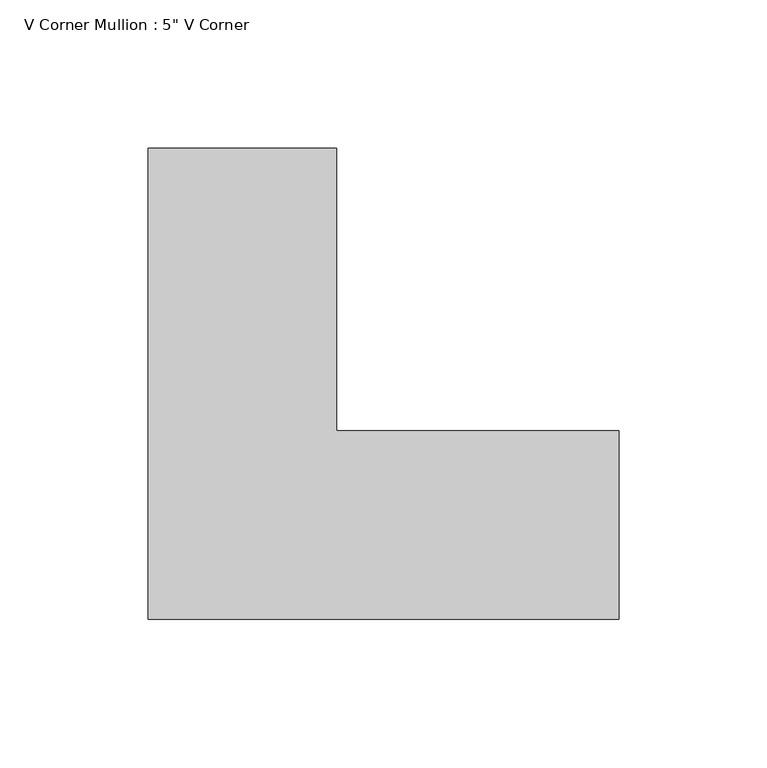
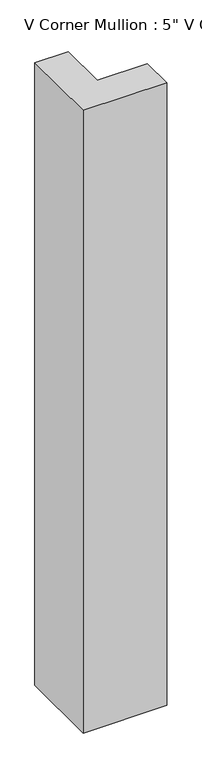
"""IFC4 building model written with IfcOpenShell, lengths in millimetres: member geometry."""

import ifcopenshell
import ifcopenshell.guid

model = None  # the IFC model being written
_history = None  # IfcOwnerHistory: only IFC2X3 demands one
_inside = {}  # id of a spatial element -> (the spatial element, [elements in it])
_under = {}  # id of a project, library or spatial element -> (it, [spatial elements below it])
_declared = {}  # id of a project -> (the project, [libraries it declares])
_typed = {}  # id of a type object -> (the type object, [elements of that type])
_made_of = {}  # id of a material, layer set ... -> (it, [elements and type objects made of it])


def new_model(schema):
    """Start an empty IFC model of exactly this schema.

    Asked for "IFC4X3", IfcOpenShell would pick the latest addendum, in which some entities
    have other attributes; the version numbers below select the first issue.
    IFC2X3 requires an IfcOwnerHistory on every rooted entity: one is made here for all.
    """
    global model, _history
    if schema == "IFC4X3":
        model = ifcopenshell.file(schema_version=(4, 3, 0, 0))
    else:
        model = ifcopenshell.file(schema=schema)
    _inside.clear()
    _under.clear()
    _declared.clear()
    _typed.clear()
    _made_of.clear()
    _history = None
    if model.schema == "IFC2X3":
        org = make("IfcOrganization", Name="unknown")
        user = make(
            "IfcPersonAndOrganization",
            ThePerson=make("IfcPerson", FamilyName="unknown"),
            TheOrganization=org,
        )
        app = make(
            "IfcApplication",
            ApplicationDeveloper=org,
            Version="unknown",
            ApplicationFullName="unknown",
            ApplicationIdentifier="unknown",
        )
        _history = make(
            "IfcOwnerHistory",
            OwningUser=user,
            OwningApplication=app,
            ChangeAction="ADDED",
            CreationDate=0,
        )
    return model


def make(cls, **values):
    """One entity of the class cls with the attributes given. An attribute that is None is left unset."""
    return model.create_entity(
        cls, **{name: value for name, value in values.items() if value is not None}
    )


def rooted(cls, **values):
    """An entity with a GlobalId (a new one), such as an element, a storey or a relation."""
    return make(cls, GlobalId=ifcopenshell.guid.new(), OwnerHistory=_history, **values)


def si_unit(unit_type, name, prefix=None):
    """IfcSIUnit, for example si_unit("LENGTHUNIT", "METRE", prefix="MILLI")."""
    return make("IfcSIUnit", UnitType=unit_type, Prefix=prefix, Name=name)


def assignment(units):
    """IfcUnitAssignment: the units of a project."""
    return None if units is None else make("IfcUnitAssignment", Units=units)


def point(xyz):
    """IfcCartesianPoint."""
    return None if xyz is None else make("IfcCartesianPoint", Coordinates=xyz)


def direction(xyz):
    """IfcDirection."""
    return None if xyz is None else make("IfcDirection", DirectionRatios=xyz)


def frame(location, z_axis=None, x_axis=None):
    """IfcAxis2Placement3D, a coordinate frame: its origin and axes. An axis left out is left unset."""
    return make(
        "IfcAxis2Placement3D",
        Location=point(location),
        Axis=direction(z_axis),
        RefDirection=direction(x_axis),
    )


def origin():
    """The frame at (0, 0, 0) with its axes left unset."""
    return frame((0.0, 0.0, 0.0))


def place(relative_to, where):
    """IfcLocalPlacement: puts the frame where relative to a parent placement (None: the world)."""
    return make(
        "IfcLocalPlacement", PlacementRelTo=relative_to, RelativePlacement=where
    )


def context(
    kind, dimensions, precision=None, world=None, true_north=None, identifier=None
):
    """IfcGeometricRepresentationContext, for example the 3D "Model" context."""
    return make(
        "IfcGeometricRepresentationContext",
        ContextIdentifier=identifier,
        ContextType=kind,
        CoordinateSpaceDimension=dimensions,
        Precision=precision,
        WorldCoordinateSystem=world,
        TrueNorth=true_north,
    )


def project(units=None, contexts=None):
    """IfcProject with its units and contexts."""
    return rooted(
        "IfcProject",
        Name="project",
        RepresentationContexts=contexts,
        UnitsInContext=assignment(units),
    )


def spatial(cls, under=None, at=None, **own):
    """A site, building, storey or space (cls), placed at a placement, below another one or the project."""
    s = rooted(cls, ObjectPlacement=at, **own)
    if under is not None:
        _under.setdefault(under.id(), (under, []))[1].append(s)
    return s


def polyline(points):
    """IfcPolyline through the points."""
    return make("IfcPolyline", Points=[point(p) for p in points])


def outline(outer, holes=None, kind="AREA"):
    """IfcArbitraryClosedProfileDef: a profile drawn as a closed curve; with holes, ...WithVoids."""
    if holes is None:
        return make("IfcArbitraryClosedProfileDef", ProfileType=kind, OuterCurve=outer)
    return make(
        "IfcArbitraryProfileDefWithVoids",
        ProfileType=kind,
        OuterCurve=outer,
        InnerCurves=holes,
    )


def extrude(swept, where, along, depth):
    """IfcExtrudedAreaSolid: the profile swept, set in the frame where, extruded along a direction by depth."""
    return make(
        "IfcExtrudedAreaSolid",
        SweptArea=swept,
        Position=where,
        ExtrudedDirection=direction(along),
        Depth=depth,
    )


def shape(context_of_items, identifier, shape_type, items):
    """IfcShapeRepresentation: the items that make up one representation, for example the "Body"."""
    return make(
        "IfcShapeRepresentation",
        ContextOfItems=context_of_items,
        RepresentationIdentifier=identifier,
        RepresentationType=shape_type,
        Items=items,
    )


def source(mapping_origin, context_of_items, identifier, shape_type, items):
    """IfcRepresentationMap: a shape defined once, which mapped items show again and again."""
    return make(
        "IfcRepresentationMap",
        MappingOrigin=mapping_origin,
        MappedRepresentation=shape(context_of_items, identifier, shape_type, items),
    )


def transform(
    local_origin,
    x_axis=None,
    y_axis=None,
    z_axis=None,
    scale=None,
    scale2=None,
    scale3=None,
    uniform=True,
):
    """IfcCartesianTransformationOperator3D, or its non-uniform kind. x_axis, y_axis, z_axis: its Axis1, 2, 3."""
    if uniform:
        return make(
            "IfcCartesianTransformationOperator3D",
            Axis1=direction(x_axis),
            Axis2=direction(y_axis),
            LocalOrigin=point(local_origin),
            Scale=scale,
            Axis3=direction(z_axis),
        )
    return make(
        "IfcCartesianTransformationOperator3DnonUniform",
        Axis1=direction(x_axis),
        Axis2=direction(y_axis),
        LocalOrigin=point(local_origin),
        Scale=scale,
        Axis3=direction(z_axis),
        Scale2=scale2,
        Scale3=scale3,
    )


def mapped(mapping_source, mapping_target):
    """IfcMappedItem: shows the shape of a source again, moved by a transform."""
    return make(
        "IfcMappedItem", MappingSource=mapping_source, MappingTarget=mapping_target
    )


def made_of(thing, what):
    """Note that an element or type object is made of a material, layer set ...; save() writes the relation."""
    if what is not None:
        _made_of.setdefault(what.id(), (what, []))[1].append(thing)
    return thing


def element(
    cls,
    number,
    at=None,
    inside=None,
    cuts=None,
    type_object=None,
    material=None,
    context=None,
    identifier="Body",
    shape_type=None,
    held_by="IfcProductDefinitionShape",
    body=None,
    shapes=None,
    **own,
):
    """One element of the class cls, such as IfcWall. Its Tag is "e" and its number.

    at: its placement. inside: the storey or other place that contains it. cuts: it is an
    opening in that element (IfcRelVoidsElement). A single representation is given by context,
    identifier, shape_type and body (its items); several are given by shapes. held_by: the class
    of the entity that holds the representations. save() writes the other relations.
    """
    e = rooted(cls, Tag="e%d" % number, ObjectPlacement=at, **own)
    if body is not None:
        shapes = [shape(context, identifier, shape_type, body)]
    if shapes is not None:
        e.Representation = make(held_by, Representations=shapes)
    if inside is not None:
        _inside.setdefault(inside.id(), (inside, []))[1].append(e)
    if cuts is not None:
        rooted(
            "IfcRelVoidsElement", RelatingBuildingElement=cuts, RelatedOpeningElement=e
        )
    if type_object is not None:
        _typed.setdefault(type_object.id(), (type_object, []))[1].append(e)
    return made_of(e, material)


def aggregate(whole, parts):
    """IfcRelAggregates: a whole, such as a stair, and the parts it consists of."""
    return rooted("IfcRelAggregates", RelatingObject=whole, RelatedObjects=parts)


def save(model, path):
    """Write the relations noted so far, then the file.

    IfcRelAggregates (storeys below a building ...), IfcRelContainedInSpatialStructure (elements
    in a storey), IfcRelDefinesByType, IfcRelAssociatesMaterial and IfcRelDeclares: one each for
    every whole, place, type object, material and project.
    """
    for whole, parts in _under.values():
        aggregate(whole, parts)
    for where, things in _inside.values():
        rooted(
            "IfcRelContainedInSpatialStructure",
            RelatedElements=things,
            RelatingStructure=where,
        )
    for kind, things in _typed.values():
        rooted("IfcRelDefinesByType", RelatedObjects=things, RelatingType=kind)
    for what, things in _made_of.values():
        rooted("IfcRelAssociatesMaterial", RelatedObjects=things, RelatingMaterial=what)
    for by, libraries in _declared.values():
        rooted("IfcRelDeclares", RelatingContext=by, RelatedDefinitions=libraries)
    model.write(path)


def member_cba7b570(model_context):
    return source(origin(), model_context, "Body", "SweptSolid", [
        extrude(outline(polyline([(63.5, -95.25), (-95.25, -95.25), (-95.25, 63.5), (-31.75, 63.5), (-31.75, -31.75), (63.5, -31.75), (63.5, -95.25)])), frame((0.0, 0.0, -1250.95), z_axis=(0.0, 0.0, 1.0), x_axis=(1.0, 0.0, 0.0)), (0.0, 0.0, 1.0), 1250.95),
    ])


if __name__ == "__main__":
    model = new_model("IFC4")
    model_context = context("Model", 3, world=origin())
    ifc_project = project(units=[si_unit("LENGTHUNIT", "METRE", prefix="MILLI")], contexts=[model_context])
    site = spatial("IfcSite", under=ifc_project)
    building = spatial("IfcBuilding", under=site)
    placement = place(None, origin())
    member_shape = member_cba7b570(model_context)
    element("IfcMember", 1, ObjectType="V Corner Mullion : 5\" V Corner", at=placement, inside=building, context=model_context, shape_type="MappedRepresentation", body=[
        mapped(member_shape, transform((0.0, 0.0, 0.0), x_axis=(1.0, 0.0, 0.0), y_axis=(0.0, 1.0, 0.0), z_axis=(0.0, 0.0, 1.0))),
    ])
    save(model, "model.ifc")

# Revit data of these elements
# Type "V Corner Mullion : 5\" V Corner"
#   built-in parameter 1007355 = 0.416667 (stored number, unit not read)
#   built-in parameter 1007354 = 0.416667 (stored number, unit not read)
#   built-in parameter 1007304 = 0.208333 (stored number, unit not read)
# Element 1 (IfcMember, "V Corner Mullion : 5\" V Corner")
#   Materials on its faces: "Aluminum"
# Materials
#   "Aluminum": class "Metal", colour RGB 247 247 247, transparency 0, Description = "Aluminum 6061", Cost = 0
